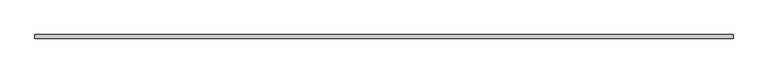
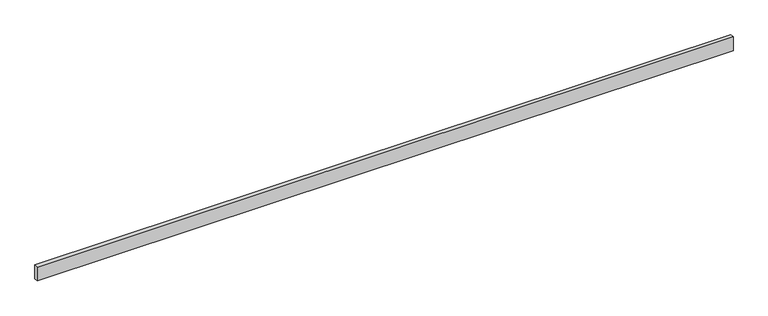
"""IFC4 building model written with IfcOpenShell, lengths in millimetres: proxy geometry, Generic Models 7:Generic Models 1:337419:Generic Models 1:337419 : Generic Models 7:Generic Models 1:337419:40 : Generic Models 7:Generic Models 1:337419:Generic Models 1:337419 : Generic Models 7:Generic Models 1:337419:301336."""

from ifc_helpers import new_model, si_unit, frame, origin, place, context, project, spatial, polyline, outline, extrude, source, transform, mapped, element, save


def generic_models_35f4e88b(model_context):
    return source(origin(), model_context, "Body", "SweptSolid", [
        extrude(outline(polyline([(596182.8367242, -536531.8913358), (596182.8367242, -536557.2913358), (591306.0367242, -536557.2913358), (591306.0367242, -536531.8913358), (596182.8367242, -536531.8913358)])), frame((0.0, 0.0, 2503.6859375), z_axis=(0.0, 0.0, 1.0), x_axis=(1.0, 0.0, 0.0)), (0.0, 0.0, 1.0), 101.6),
    ])


if __name__ == "__main__":
    model = new_model("IFC4")
    model_context = context("Model", 3, world=origin())
    ifc_project = project(units=[si_unit("LENGTHUNIT", "METRE", prefix="MILLI")], contexts=[model_context])
    site = spatial("IfcSite", under=ifc_project)
    building = spatial("IfcBuilding", under=site)
    placement = place(None, origin())
    generic_models_shape = generic_models_35f4e88b(model_context)
    element("IfcBuildingElementProxy", 1, Name="Generic Models 7:Generic Models 1:337419:Generic Models 1:337419 : Generic Models 7:Generic Models 1:337419:40 : Generic Models 7:Generic Models 1:337419:Generic Models 1:337419 : Generic Models 7:Generic Models 1:337419:301336", ObjectType="Generic Models 7:Generic Models 1:337419:Generic Models 1:337419 : Generic Models 7:Generic Models 1:337419:40 : Generic Models 7:Generic Models 1:337419:Generic Models 1:337419 : Generic Models 7:Generic Models 1:337419:301336", at=placement, inside=building, context=model_context, shape_type="MappedRepresentation", body=[
        mapped(generic_models_shape, transform((0.0, 0.0, 0.0), x_axis=(1.0, 0.0, 0.0), y_axis=(0.0, 1.0, 0.0), z_axis=(0.0, 0.0, 1.0))),
    ])
    save(model, "model.ifc")

# Revit data of these elements
# Type "Generic Models 7:Generic Models 1:337419:Generic Models 1:337419 : Generic Models 7:Generic Models 1:337419:40 : Generic Models 7:Generic Models 1:337419:Generic Models 1:337419 : Generic Models 7:Generic Models 1:337419:301336"
#   NameOverride = "Generic Models 7:Generic Models 1:337419:Generic Models 1:337419 : Generic Models 7:Generic Models 1:337419:301336"
#   ObjectTypeOverride = "Generic Models 1:337419 : Generic Models 7:Generic Models 1:337419"
#   Reference = "Generic Models 1"
#   Tag = "301336"
# Element 1 (IfcBuildingElementProxy, "Generic Models 7:Generic Models 1:337419:Generic Models 1:337419 : Generic Models 7:Generic Models 1:337419:40 : Generic Models 7:Generic Models 1:337419:Generic Models 1:337419 : Generic Models 7:Generic Models 1:337419:301336")
#   Materials on its faces: "RIGID INSULATION AT GIRTS/JAMB - (CLASS A FLAME SPREAD)"
# Materials
#   "RIGID INSULATION AT GIRTS/JAMB - (CLASS A FLAME SPREAD)": class "Unassigned", colour RGB 205 188 106, transparency 0, Cost = 0
